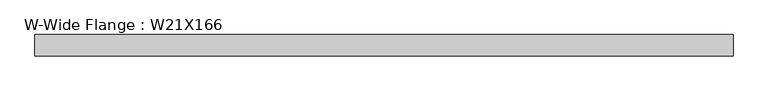
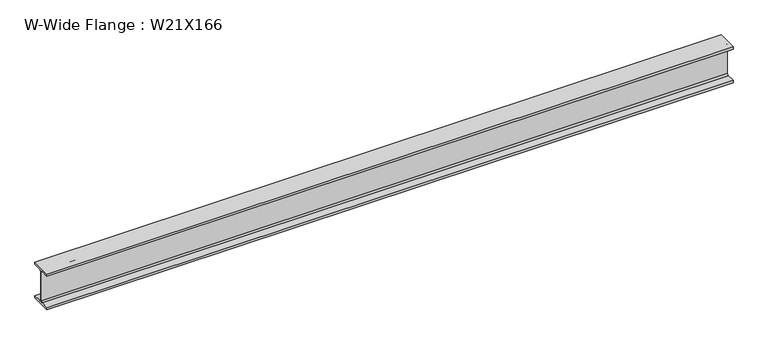
"""IFC4 building model written with IfcOpenShell, lengths in millimetres: beam geometry, W-Wide Flange : W21X166."""

from ifc_helpers import new_model, si_unit, point, frame, frame_2d, origin, place, context, project, spatial, polyline, circle_curve, trimmed, segment, composite_curve, outline, extrude, source, transform, mapped, element, save


def w_wide_flange_w21x166_efd61159(model_context):
    return source(origin(), model_context, "Body", "SweptSolid", [
        extrude(outline(composite_curve([segment(polyline([(157.48, -251.206), (157.48, -285.75), (-157.48, -285.75), (-157.48, -251.206), (-32.131, -251.206)]), True, "CONTINUOUS"), segment(trimmed(circle_curve(frame_2d((-32.131, -228.6)), 22.606), [point((-32.131, -251.206))], [point((-9.525, -228.6))], True, "CARTESIAN"), True, "CONTINUOUS"), segment(polyline([(-9.525, -228.6), (-9.525, 228.6)]), True, "CONTINUOUS"), segment(trimmed(circle_curve(frame_2d((-32.131, 228.6)), 22.606), [point((-9.525, 228.6))], [point((-32.131, 251.206))], True, "CARTESIAN"), True, "CONTINUOUS"), segment(polyline([(-32.131, 251.206), (-157.48, 251.206), (-157.48, 285.75), (157.48, 285.75), (157.48, 251.206), (32.131, 251.206)]), True, "CONTINUOUS"), segment(trimmed(circle_curve(frame_2d((32.131, 228.6)), 22.606), [point((32.131, 251.206))], [point((9.525, 228.6))], True, "CARTESIAN"), True, "CONTINUOUS"), segment(polyline([(9.525, 228.6), (9.525, -228.6)]), True, "CONTINUOUS"), segment(trimmed(circle_curve(frame_2d((32.131, -228.6)), 22.606), [point((9.525, -228.6))], [point((32.131, -251.206))], True, "CARTESIAN"), True, "CONTINUOUS"), segment(polyline([(32.131, -251.206), (157.48, -251.206)]), True, "CONTINUOUS")], self_intersect=False)), frame((-5139.3101369, 0.0, 0.0), z_axis=(1.0, 0.0, 0.0), x_axis=(0.0, 1.0, 0.0)), (0.0, 0.0, 1.0), 10368.5713579),
    ])


if __name__ == "__main__":
    model = new_model("IFC4")
    model_context = context("Model", 3, world=origin())
    ifc_project = project(units=[si_unit("LENGTHUNIT", "METRE", prefix="MILLI")], contexts=[model_context])
    site = spatial("IfcSite", under=ifc_project)
    building = spatial("IfcBuilding", under=site)
    placement = place(None, origin())
    w_wide_flange_w21x166_shape = w_wide_flange_w21x166_efd61159(model_context)
    element("IfcBeam", 1, ObjectType="W-Wide Flange : W21X166", at=placement, inside=building, context=model_context, shape_type="MappedRepresentation", body=[
        mapped(w_wide_flange_w21x166_shape, transform((0.0, 0.0, 0.0), x_axis=(1.0, 0.0, 0.0), y_axis=(0.0, 1.0, 0.0), z_axis=(0.0, 0.0, 1.0))),
    ])
    save(model, "model.ifc")

# Revit data of these elements
# Type "W-Wide Flange : W21X166"
#   Assembly Code = "B10"
#   W = 166
#   Length [instance default] = 5' - 0"
#   bf = 1' - 0.4"
#   d = 1' - 10 1/2"
#   k = 0' - 2 1/4"
#   k2 = 0' - 0.89"
#   tf = 0' - 1.36"
#   tw = 0' - 0 3/4"
#   A = 0.338889 SF
#   Structural Material [instance default] = Steel ASTM A992
# Element 1 (IfcBeam, "W-Wide Flange : W21X166")
#   Structural Material = Steel
#   Materials on its faces: "Steel"
# Materials
#   "Steel ASTM A992": class "Metal", colour RGB 199 199 199, transparency 0, Description = "Structural steel 50ksi", Cost = 0
#   "Steel": class "Metal", colour RGB 118 118 114, transparency 0, Description = "Steel, mill finish", Cost = 0
